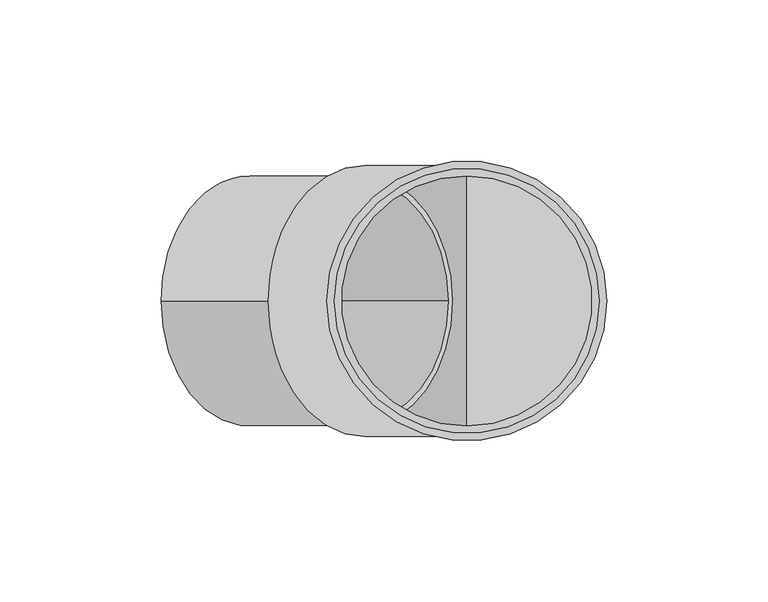
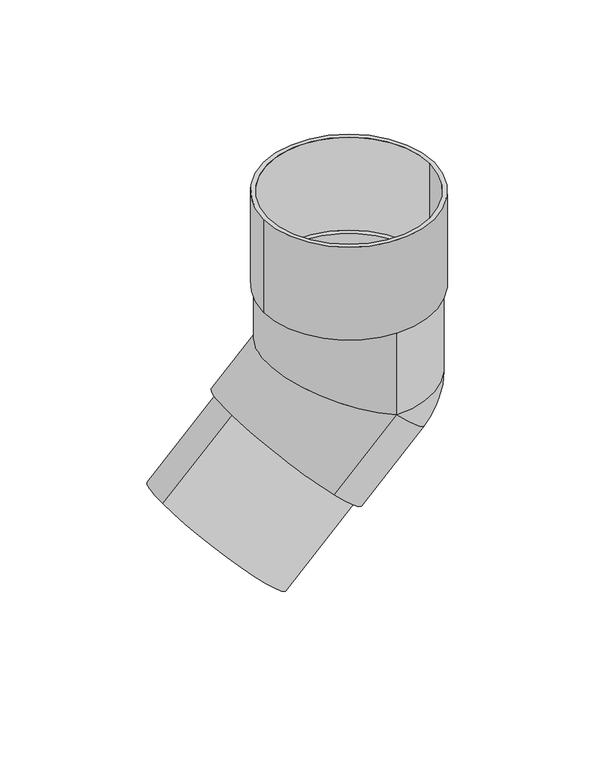
"""IFC4 building model written with IfcOpenShell, lengths in millimetres: proxy geometry, ⇲ Колено трубы 135 : ⇲ Колено трубы 135."""

from ifc_helpers import new_model, si_unit, point, frame, origin, origin_with_axes, place, context, project, spatial, polyline, circle_curve, ellipse_curve, trimmed, source, transform, mapped, element, save
from ifc_brep_helpers import plane_surface, cylinder_surface, revolved_surface, advanced_brep


def generic_models_f3c7a8e8(model_context):
    return source(origin(), model_context, "Body", "AdvancedBrep", [
        advanced_brep(
        [(41.1, 0.0, -50.0), (-41.1, 0.0, -50.0), (0.0, -38.8, -50.0), (0.0, 38.8, -50.0), (0.0, -42.0, -50.0), (0.0, 42.0, -50.0), (0.0, 42.0, -95.0), (0.0, -42.0, -95.0), (42.0, 0.0, -95.0), (0.0, 38.8, -95.0), (0.0, -38.8, -95.0), (-31.8198052, -42.0, -126.8198052), (-31.8198052, 42.0, -126.8198052), (-59.2555483, 0.0, -99.384062), (-31.8198052, -38.8, -126.8198052), (-4.384062, 0.0, -154.2555483), (-31.8198052, 38.8, -126.8198052), (29.6984848, 0.0, -124.6984848), (-31.8198052, 38.8, -126.8198052), (-4.384062, 0.0, -154.2555483), (-31.8198052, -38.8, -126.8198052), (-59.2555483, 0.0, -99.384062), (-43.4, 0.0, 0.0), (43.4, 0.0, 0.0), (-41.1, 0.0, 0.0), (41.1, 0.0, 0.0), (-43.4, 0.0, -50.0), (43.4, 0.0, -50.0), (-57.8413347, 0.0, -100.7982756), (-5.7982756, 0.0, -152.8413347), (-94.787868, 0.0, -134.9163817), (-39.9163817, 0.0, -189.787868), (-93.3736544, 0.0, -136.3305953), (-41.3305953, 0.0, -188.3736544)],
        [
            (0, 1, circle_curve(frame((0.0, 0.0, -50.0), z_axis=(0.0, 0.0, 1.0), x_axis=(1.0, 0.0, 0.0)), 41.1)),
            (1, 0, circle_curve(frame((0.0, 0.0, -50.0), z_axis=(0.0, 0.0, 1.0), x_axis=(1.0, 0.0, 0.0)), 41.1)),
            (2, 3, circle_curve(frame((0.0, 0.0, -50.0), z_axis=(0.0, 0.0, -1.0), x_axis=(0.0, 1.0, 0.0)), 38.8)),
            (3, 2, circle_curve(frame((0.0, 0.0, -50.0), z_axis=(0.0, 0.0, -1.0), x_axis=(0.0, 1.0, 0.0)), 38.8)),
            (4, 5, circle_curve(frame((0.0, 0.0, -50.0), z_axis=(0.0, 0.0, -1.0), x_axis=(0.0, 1.0, 0.0)), 42.0)),
            (5, 6),
            (6, 7, ellipse_curve(frame((0.0, 0.0, -95.0), z_axis=(0.38268343236509084, 0.0, 0.9238795325112863), x_axis=(-0.9238795325112863, 0.0, 0.38268343236509084)), 45.4604724, 42.0)),
            (7, 4),
            (7, 8, circle_curve(frame((0.0, 0.0, -95.0), z_axis=(0.0, 0.0, 1.0), x_axis=(0.0, 1.0, 0.0)), 42.0)),
            (8, 6, circle_curve(frame((0.0, 0.0, -95.0), z_axis=(0.0, 0.0, 1.0), x_axis=(0.0, 1.0, 0.0)), 42.0)),
            (5, 4, circle_curve(frame((0.0, 0.0, -50.0), z_axis=(0.0, 0.0, -1.0), x_axis=(0.0, 1.0, 0.0)), 42.0)),
            (3, 9),
            (9, 10, circle_curve(frame((0.0, 0.0, -95.0), z_axis=(0.0, 0.0, -1.0), x_axis=(0.0, 1.0, 0.0)), 38.8)),
            (10, 2),
            (10, 9, ellipse_curve(frame((0.0, 0.0, -95.0), z_axis=(-0.38268343236509084, 0.0, -0.9238795325112863), x_axis=(0.9238795325112863, 0.0, -0.38268343236509084)), 41.9968174, 38.8)),
            (11, 12, circle_curve(frame((-31.8198052, 0.0, -126.8198052), z_axis=(-0.7071067811865479, 0.0, -0.7071067811865471), x_axis=(0.0, 1.0, 0.0)), 42.0)),
            (12, 11, circle_curve(frame((-31.8198052, 0.0, -126.8198052), z_axis=(-0.7071067811865479, 0.0, -0.7071067811865471), x_axis=(0.0, 1.0, 0.0)), 42.0)),
            (13, 14, circle_curve(frame((-31.8198052, 0.0, -126.8198052), z_axis=(0.7071067811865457, 0.0, 0.7071067811865495), x_axis=(0.7071067811865495, 0.0, -0.7071067811865457)), 38.8)),
            (14, 15, circle_curve(frame((-31.8198052, 0.0, -126.8198052), z_axis=(0.7071067811865457, 0.0, 0.7071067811865495), x_axis=(0.7071067811865495, 0.0, -0.7071067811865457)), 38.8)),
            (15, 16, circle_curve(frame((-31.8198052, 0.0, -126.8198052), z_axis=(0.7071067811865457, 0.0, 0.7071067811865495), x_axis=(0.7071067811865495, 0.0, -0.7071067811865457)), 38.8)),
            (16, 13, circle_curve(frame((-31.8198052, 0.0, -126.8198052), z_axis=(0.7071067811865457, 0.0, 0.7071067811865495), x_axis=(0.7071067811865495, 0.0, -0.7071067811865457)), 38.8)),
            (6, 12),
            (11, 7),
            (6, 17, circle_curve(frame((0.0, 0.0, -95.0), z_axis=(-0.7071067811865479, 0.0, -0.7071067811865471), x_axis=(0.0, 1.0, 0.0)), 42.0)),
            (17, 7, circle_curve(frame((0.0, 0.0, -95.0), z_axis=(-0.7071067811865479, 0.0, -0.7071067811865471), x_axis=(0.0, 1.0, 0.0)), 42.0)),
            (10, 9, circle_curve(frame((0.0, 0.0, -95.0), z_axis=(0.7071067811865479, 0.0, 0.7071067811865471), x_axis=(0.0, 1.0, 0.0)), 38.8)),
            (9, 18),
            (18, 19, circle_curve(frame((-31.8198052, 0.0, -126.8198052), z_axis=(-0.7071067811865479, 0.0, -0.7071067811865471), x_axis=(0.0, 1.0, 0.0)), 38.8)),
            (19, 20, circle_curve(frame((-31.8198052, 0.0, -126.8198052), z_axis=(-0.7071067811865479, 0.0, -0.7071067811865471), x_axis=(0.0, 1.0, 0.0)), 38.8)),
            (20, 10),
            (20, 21, circle_curve(frame((-31.8198052, 0.0, -126.8198052), z_axis=(-0.7071067811865479, 0.0, -0.7071067811865471), x_axis=(0.0, 1.0, 0.0)), 38.8)),
            (21, 18, circle_curve(frame((-31.8198052, 0.0, -126.8198052), z_axis=(-0.7071067811865479, 0.0, -0.7071067811865471), x_axis=(0.0, 1.0, 0.0)), 38.8)),
            (9, 10),
            (8, 17, circle_curve(frame((0.0, 0.0, -95.0), z_axis=(0.0, 1.0, 0.0), x_axis=(1.0, 0.0, 0.0)), 42.0)),
            (22, 23, circle_curve(origin_with_axes(), 43.4)),
            (23, 22, circle_curve(origin_with_axes(), 43.4)),
            (24, 25, circle_curve(frame((0.0, 0.0, 0.0), z_axis=(0.0, 0.0, -1.0), x_axis=(1.0, 0.0, 0.0)), 41.1)),
            (25, 24, circle_curve(frame((0.0, 0.0, 0.0), z_axis=(0.0, 0.0, -1.0), x_axis=(1.0, 0.0, 0.0)), 41.1)),
            (26, 27, circle_curve(frame((0.0, 0.0, -50.0), z_axis=(0.0, 0.0, -1.0), x_axis=(1.0, 0.0, 0.0)), 43.4)),
            (27, 26, circle_curve(frame((0.0, 0.0, -50.0), z_axis=(0.0, 0.0, -1.0), x_axis=(1.0, 0.0, 0.0)), 43.4)),
            (25, 0),
            (1, 24),
            (23, 27),
            (26, 22),
            (28, 29, circle_curve(frame((-31.8198052, 0.0, -126.8198052), z_axis=(-0.7071067811865457, 0.0, -0.7071067811865495), x_axis=(0.7071067811865495, 0.0, -0.7071067811865457)), 36.8)),
            (29, 28, circle_curve(frame((-31.8198052, 0.0, -126.8198052), z_axis=(-0.7071067811865457, 0.0, -0.7071067811865495), x_axis=(0.7071067811865495, 0.0, -0.7071067811865457)), 36.8)),
            (30, 31, circle_curve(frame((-67.3521249, 0.0, -162.3521249), z_axis=(-0.7071067811865457, 0.0, -0.7071067811865495), x_axis=(0.7071067811865495, 0.0, -0.7071067811865457)), 38.8)),
            (31, 30, circle_curve(frame((-67.3521249, 0.0, -162.3521249), z_axis=(-0.7071067811865457, 0.0, -0.7071067811865495), x_axis=(0.7071067811865495, 0.0, -0.7071067811865457)), 38.8)),
            (32, 33, circle_curve(frame((-67.3521249, 0.0, -162.3521249), z_axis=(0.7071067811865457, 0.0, 0.7071067811865495), x_axis=(0.7071067811865495, 0.0, -0.7071067811865457)), 36.8)),
            (33, 32, circle_curve(frame((-67.3521249, 0.0, -162.3521249), z_axis=(0.7071067811865457, 0.0, 0.7071067811865495), x_axis=(0.7071067811865495, 0.0, -0.7071067811865457)), 36.8)),
            (30, 13),
            (15, 31),
            (29, 33),
            (32, 28),
        ],
        [
            plane_surface(frame((0.0, 0.0, -50.0), z_axis=(0.0, 0.0, 1.0), x_axis=(0.0, 1.0, 0.0))),
            cylinder_surface(frame((0.0, 0.0, -50.0), z_axis=(0.0, 0.0, 1.0), x_axis=(0.0, 1.0, 0.0)), 42.0),
            revolved_surface(polyline([(0.0, 38.8, -95.0), (0.0, 38.8, -50.0)]), (0.0, 0.0, -50.0), (0.0, 0.0, -1.0)),
            revolved_surface(polyline([(0.0, 38.8, -111.07148623104197), (0.0, 38.8, -50.0)]), (0.0, 0.0, -50.0), (0.0, 0.0, -1.0)),
            plane_surface(frame((-31.8198052, 0.0, -126.8198052), z_axis=(-0.7071067811865479, 0.0, -0.7071067811865471), x_axis=(0.0, 1.0, 0.0))),
            cylinder_surface(frame((0.0, 0.0, -95.0), z_axis=(0.7071067811865479, 0.0, 0.7071067811865471), x_axis=(0.0, 1.0, 0.0)), 42.0),
            revolved_surface(polyline([(-31.81980520000002, 38.8, -126.81980519999999), (0.0, 38.8, -95.0)]), (0.0, 0.0, -95.0), (-0.7071067811865479, 0.0, -0.7071067811865471)),
            revolved_surface(polyline([(-31.81980520000002, 38.8, -126.81980519999999), (11.364256897715961, 38.8, -83.63574310228405)]), (0.0, 0.0, -95.0), (-0.7071067811865479, 0.0, -0.7071067811865471)),
            plane_surface(frame((0.0, -2000.0, -95.0), z_axis=(0.0, 0.0, 1.0), x_axis=(1.0, 0.0, 0.0))),
            plane_surface(frame((0.0, -2000.0, -95.0), z_axis=(-0.707106781186547, 0.0, -0.7071067811865482), x_axis=(0.7071067811865482, 0.0, -0.707106781186547))),
            revolved_surface(trimmed(ellipse_curve(frame((0.0, 0.0, -95.0), z_axis=(0.0, 0.0, -1.0), x_axis=(1.0, 0.0, 0.0)), 42.0, 42.0), [point((0.0, 42.0, -95.0))], [point((42.0, 0.0, -95.0))], True, "CARTESIAN"), (0.0, -2000.0, -95.0), (0.0, -1.0, 0.0)),
            revolved_surface(trimmed(ellipse_curve(frame((0.0, 0.0, -95.0), z_axis=(0.0, 0.0, -1.0), x_axis=(1.0, 0.0, 0.0)), 42.0, 42.0), [point((42.0, 0.0, -95.0))], [point((0.0, -42.0, -95.0))], True, "CARTESIAN"), (0.0, -2000.0, -95.0), (0.0, -1.0, 0.0)),
            plane_surface(frame((41.1, 0.0, 0.0), z_axis=(0.0, 0.0, 1.0), x_axis=(0.0, 1.0, 0.0))),
            plane_surface(frame((41.1, 0.0, -50.0), z_axis=(0.0, 0.0, -1.0), x_axis=(0.0, -1.0, 0.0))),
            revolved_surface(polyline([(41.1, 0.0, -50.0), (41.1, 0.0, 0.0)]), (0.0, 0.0, -50.0), (0.0, 0.0, -1.0)),
            cylinder_surface(origin_with_axes(), 43.4),
            plane_surface(frame((-31.8198052, 0.0, -126.8198052), z_axis=(0.7071067811865457, 0.0, 0.7071067811865495), x_axis=(0.0, 1.0, 0.0))),
            plane_surface(frame((-67.3521249, 0.0, -162.3521249), z_axis=(-0.7071067811865457, 0.0, -0.7071067811865495), x_axis=(0.0, 1.0, 0.0))),
            cylinder_surface(frame((-31.8198052, 0.0, -126.8198052), z_axis=(0.7071067811865457, 0.0, 0.7071067811865495), x_axis=(0.7071067811865495, 0.0, -0.7071067811865457)), 38.8),
            revolved_surface(polyline([(-41.330595352334896, 0.0, -188.373654447665), (-5.7982756023349085, 0.0, -152.84133469766482)]), (-31.8198052, 0.0, -126.8198052), (-0.7071067811865457, 0.0, -0.7071067811865495)),
        ],
        [
            (0, [[1, 2], [3, 4]]),
            (1, [[5, 6, 7, 8]]),
            (1, [[9, 10, -6, 11, -8]]),
            (2, [[12, 13, 14, -4]]),
            (3, [[-14, 15, -12, -3]]),
            (4, [[16, 17], [18, 19, 20, 21]]),
            (5, [[22, -16, 23, -7]]),
            (5, [[-22, 24, 25, -23, -17]]),
            (6, [[26, 27, 28, 29, 30]]),
            (7, [[-30, 31, 32, -27, -15]]),
            (8, [[-13, 33]]),
            (9, [[-26, -33]]),
            (10, [[-24, -10, 34]]),
            (11, [[-9, -25, -34]]),
            (12, [[35, 36], [37, 38]]),
            (13, [[39, 40], [-11, -5]]),
            (14, [[41, -2, 42, -38]]),
            (14, [[-42, -1, -41, -37]]),
            (15, [[43, -39, 44, -36]]),
            (15, [[-44, -40, -43, -35]]),
            (16, [[-28, -32, -31, -29], [45, 46]]),
            (17, [[47, 48], [49, 50]]),
            (18, [[51, -21, -20, 52, -47]]),
            (18, [[-52, -19, -18, -51, -48]]),
            (19, [[53, -49, 54, -46]]),
            (19, [[-54, -50, -53, -45]]),
        ],
    ),
    ])


if __name__ == "__main__":
    model = new_model("IFC4")
    model_context = context("Model", 3, world=origin())
    ifc_project = project(units=[si_unit("LENGTHUNIT", "METRE", prefix="MILLI")], contexts=[model_context])
    site = spatial("IfcSite", under=ifc_project)
    building = spatial("IfcBuilding", under=site)
    placement = place(None, origin())
    generic_models_shape = generic_models_f3c7a8e8(model_context)
    element("IfcBuildingElementProxy", 1, Name="⇲ Колено трубы 135 : ⇲ Колено трубы 135", ObjectType="⇲ Колено трубы 135 : ⇲ Колено трубы 135", at=placement, inside=building, context=model_context, shape_type="MappedRepresentation", body=[
        mapped(generic_models_shape, transform((0.0, 0.0, 0.0), x_axis=(1.0, 0.0, 0.0), y_axis=(0.0, 1.0, 0.0), z_axis=(0.0, 0.0, 1.0))),
    ])
    save(model, "model.ifc")

# Revit data of these elements
# Type "⇲ Колено трубы 135 : ⇲ Колено трубы 135"
#   Description = "Предназначено для изменения направления стока по трубе. Также применяется для обхода архитектурных элементов\r\nфасада"
#   Manufacturer = "ТехноНИКОЛЬ"
#   Model = "Комплектующие к водосточным системам"
#   URL = "https://tn-vodostok.ru/catalog/pvh/"
#   ADSK_Обозначение = "ТехноНИКОЛЬ"
#   ADSK_Наименование краткое = "Колено 135°"
#   ADSK_Наименование = "Колено трубы 135°"
#   ADSK_Масса_Текст = ""
#   ADSK_Марка = ""
#   ADSK_Код изделия = ""
#   ADSK_Завод-изготовитель = "ТехноНИКОЛЬ"
#   ADSK_Единица измерения = "шт."
#   ADSK_Группирование = "Комплектующие к водосточным системам"
#   ADSK_URL страницы изделия = "https://tn-vodostok.ru/catalog/pvh/"
#   ADSK_URL документации изделия = "https://tn-vodostok.ru/upload/iblock/c42/c427963cb77eb5c3c51f0cfb870e9e52.pdf"
#   Угол поворота хомута [instance default] = 0.00°
#   ADSK_Размер_Ширина = 143.3 mm
#   ADSK_Размер_Диаметр = 82.2 mm
#   ADSK_Размер_Высота = 190 mm
#   ADSK_Количество = 1
#   ADSK_Материал [instance default] = TN_Пластик_Коричневый_RAL8019
#   Default Elevation = 0
# Element 1 (IfcBuildingElementProxy, "⇲ Колено трубы 135 : ⇲ Колено трубы 135")
#   Materials on its faces: "TN_Пластик_Коричневый_RAL8019"
# Materials
#   "TN_Пластик_Коричневый_RAL8019": class "Типовые", colour RGB 61 54 53, transparency 0, Cost = 0
